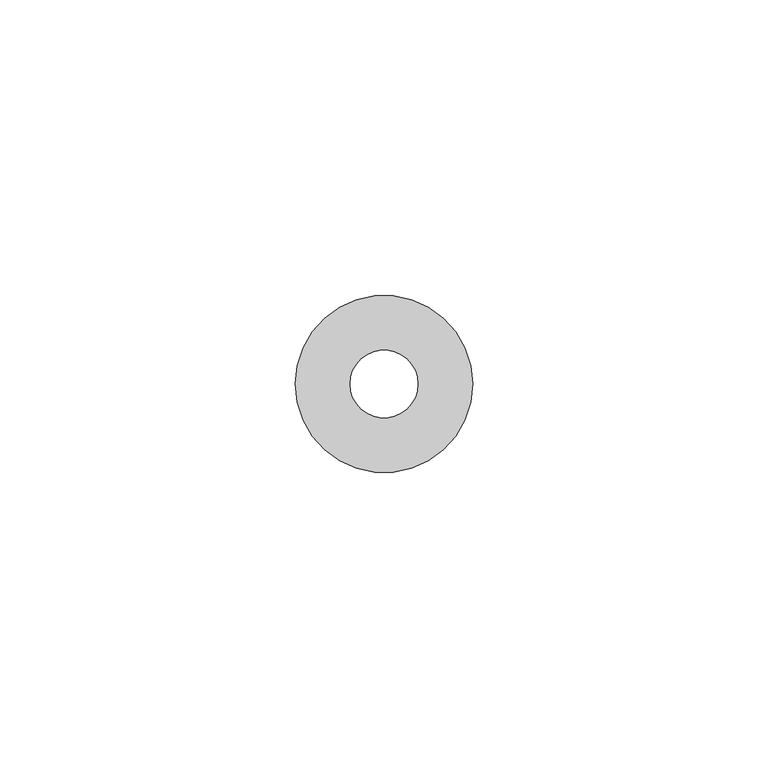
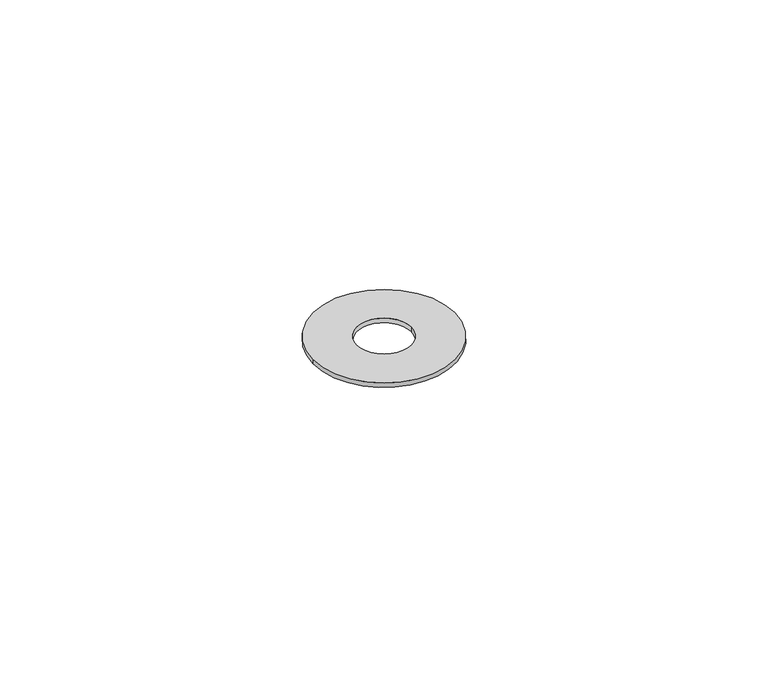
"""IFC4 building model written with IfcOpenShell, lengths in millimetres: proxy geometry, TN_Шайба увеличенная : Шайба увеличенная M10 D40 3F."""

from ifc_helpers import new_model, si_unit, point, frame, origin, origin_2d, place, context, project, spatial, circle_curve, trimmed, segment, composite_curve, outline, extrude, source, transform, mapped, element, save


def generic_models_5c0ffc5b(model_context):
    return source(origin(), model_context, "Body", "SweptSolid", [
        extrude(outline(composite_curve([segment(trimmed(circle_curve(origin_2d(), 15.0), [point((-15.0, 0.0))], [point((15.0, 0.0))], False, "CARTESIAN"), True, "CONTINUOUS"), segment(trimmed(circle_curve(origin_2d(), 15.0), [point((15.0, 0.0))], [point((-15.0, 0.0))], False, "CARTESIAN"), True, "CONTINUOUS")], self_intersect=False), holes=[composite_curve([segment(trimmed(circle_curve(origin_2d(), 5.75), [point((-5.75, 0.0))], [point((5.75, 0.0))], True, "CARTESIAN"), True, "CONTINUOUS"), segment(trimmed(circle_curve(origin_2d(), 5.75), [point((5.75, 0.0))], [point((-5.75, 0.0))], True, "CARTESIAN"), True, "CONTINUOUS")], self_intersect=False)]), frame((0.0, 0.0, -1.0), z_axis=(0.0, 0.0, 1.0), x_axis=(1.0, 0.0, 0.0)), (0.0, 0.0, 1.0), 1.0),
    ])


if __name__ == "__main__":
    model = new_model("IFC4")
    model_context = context("Model", 3, world=origin())
    ifc_project = project(units=[si_unit("LENGTHUNIT", "METRE", prefix="MILLI")], contexts=[model_context])
    site = spatial("IfcSite", under=ifc_project)
    building = spatial("IfcBuilding", under=site)
    placement = place(None, origin())
    generic_models_shape = generic_models_5c0ffc5b(model_context)
    element("IfcBuildingElementProxy", 1, Name="TN_Шайба увеличенная : Шайба увеличенная M10 D40 3F", ObjectType="TN_Шайба увеличенная : Шайба увеличенная M10 D40 3F", at=placement, inside=building, context=model_context, shape_type="MappedRepresentation", body=[
        mapped(generic_models_shape, transform((0.0, 0.0, 0.0), x_axis=(1.0, 0.0, 0.0), y_axis=(0.0, 1.0, 0.0), z_axis=(0.0, 0.0, 1.0))),
    ])
    save(model, "model.ifc")

# Revit data of these elements
# Type "TN_Шайба увеличенная : Шайба увеличенная M10 D40 3F"
#   Description = "Шайбы применяются для обеспечения эффективной фиксации креплений. Шайба в соединении создает большую опорную площадь, распределяет нагрузку и может служить для предотвращения самоотвинчивания крепежных изделий."
#   Manufacturer = "ТехноНИКОЛЬ"
#   Model = "Комплектующие к опорам"
#   URL = "https://nav.tn.ru/knowledge-base/polimernye-membrany/opory-pod-oborudovanie-na-ploskoy-krovle/?sphrase_id=266812"
#   ADSK_Обозначение = "ТехноНИКОЛЬ"
#   ADSK_Наименование краткое = "M10 D40 3F"
#   ADSK_Наименование = "Шайба увеличенная M10 D40 3F"
#   ADSK_Масса_Текст = ""
#   ADSK_Марка = "M10 D40 3F"
#   ADSK_Код изделия = "660822"
#   ADSK_Завод-изготовитель = "ТехноНИКОЛЬ"
#   ADSK_Единица измерения = "шт."
#   ADSK_Группирование = "Комплектующие к опорам"
#   ADSK_URL страницы изделия = "https://nav.tn.ru/knowledge-base/polimernye-membrany/opory-pod-oborudovanie-na-ploskoy-krovle/?sphrase_id=266812"
#   ADSK_URL документации изделия = ""
#   ADSK_Количество = 1
#   ADSK_Материал = TN_СтальГальванизированная_Серый
#   Default Elevation = 0
# Element 1 (IfcBuildingElementProxy, "TN_Шайба увеличенная : Шайба увеличенная M10 D40 3F")
#   Materials on its faces: "TN_СтальГальванизированная_Серый"
# Materials
#   "TN_СтальГальванизированная_Серый": class "Типовые", colour RGB 206 210 213, transparency 0, Cost = 0
